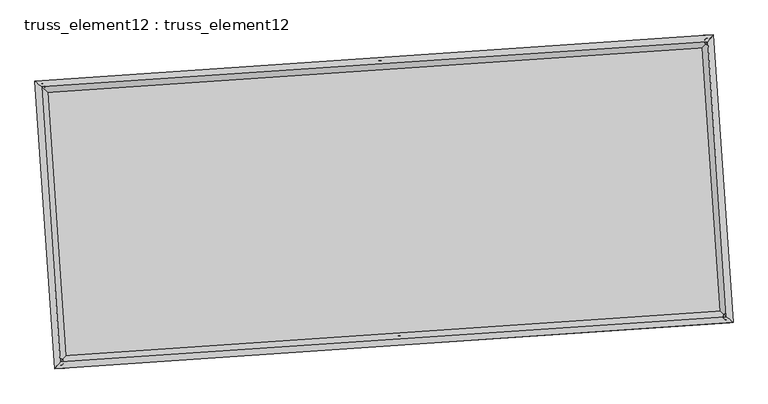
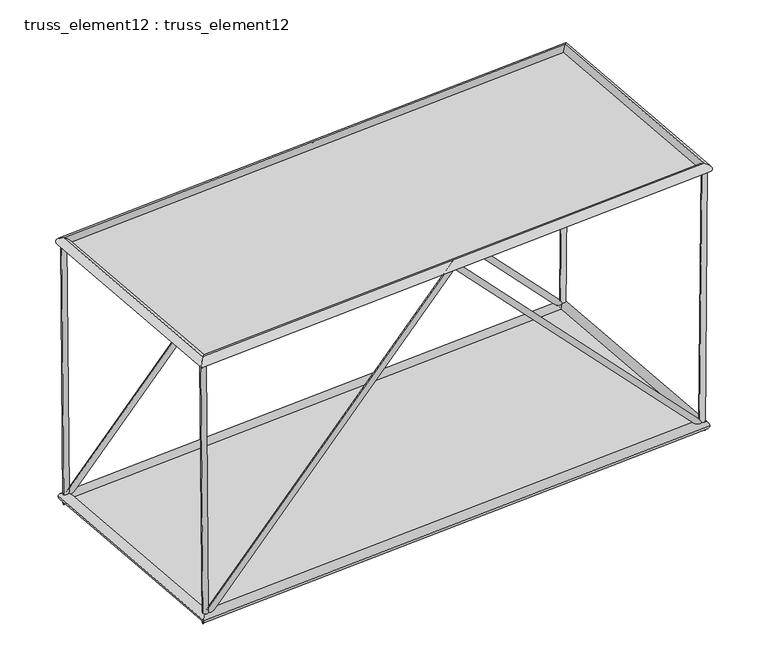
"""IFC4 building model written with IfcOpenShell, lengths in millimetres: plate geometry, truss_element12 : truss_element12."""

from ifc_helpers import new_model, si_unit, frame, origin, origin_with_axes, place, context, project, spatial, polyline, circle_curve, ellipse_curve, outline, extrude, source, transform, mapped, element, save
from ifc_brep_helpers import plane_surface, cylinder_surface, advanced_brep


def truss_element12_truss_element12_a0b56646(model_context):
    return source(origin(), model_context, "Body", "SolidModel", [
        advanced_brep(
        [(-3711.0240607, 2273.081801, 5000.2475381), (-3810.123175, 2259.720815, 4999.3258018), (-3666.0735064, 2276.1468084, 123.0270128), (-3762.9133765, 2262.9398717, -123.0270128), (1063.3254717, 2598.6265466, 5071.9126371), (1063.7795579, 2592.0537149, 4927.6678823), (5793.4932269, 2921.1587048, 123.0325352), (5891.2677501, 2921.2217837, -123.0325352), (5837.6808151, 2924.1716885, 5000.2468963), (5937.6764799, 2924.3862186, 4999.3408025)],
        [
            (0, 1, circle_curve(frame((-3760.5736179, 2266.401308, 4999.7866699), z_axis=(-0.009216035288574901, -0.0006284064129009009, 0.9999573339892758), x_axis=(-0.1336099520450236, 0.9910338088636684, -0.000608607998935612)), 50.0)),
            (1, 0, circle_curve(frame((-3760.5736179, 2266.401308, 4999.7866699), z_axis=(-0.009216035288574901, -0.0006284064129009009, 0.9999573339892758), x_axis=(-0.1336099520450236, 0.9910338088636684, -0.000608607998935612)), 50.0)),
            (0, 2),
            (2, 3, ellipse_curve(frame((-3714.4934414, 2269.54334, 0.0), z_axis=(-0.9275008521416528, -0.06324275734672205, 0.3684325215282871), x_axis=(0.36757900930277176, 0.025063815345724785, 0.9296544933900488)), 132.6244381, 50.0)),
            (3, 1),
            (3, 2, ellipse_curve(frame((-3714.4934414, 2269.54334, 0.0), z_axis=(-0.9275008521416528, -0.06324275734672205, 0.3684325215282871), x_axis=(0.36757900930277176, 0.025063815345724785, 0.9296544933900488)), 132.6244381, 50.0)),
            (2, 4),
            (4, 5, ellipse_curve(frame((1063.5525148, 2595.3401308, 4999.7902597), z_axis=(-0.9976833952413824, -0.06802823817186877, -4.08761425662505e-05), x_axis=(4.0781448733720234e-05, 2.7807319673914647e-06, -0.9999999991645705)), 72.2794243, 50.0)),
            (5, 3),
            (5, 4, ellipse_curve(frame((1063.5525148, 2595.3401308, 4999.7902597), z_axis=(-0.9976833952413824, -0.06802823817186877, -4.08761425662505e-05), x_axis=(4.0781448733720234e-05, 2.7807319673914647e-06, -0.9999999991645705)), 72.2794243, 50.0)),
            (4, 6),
            (6, 7, ellipse_curve(frame((5842.3804885, 2921.1902443, 0.0), z_axis=(-0.9274570070583223, -0.06323976771715853, -0.36854339206869385), x_axis=(-0.3676896230000489, -0.025071357673265647, 0.9296105464991785)), 132.6366613, 50.0)),
            (7, 5),
            (7, 6, ellipse_curve(frame((5842.3804885, 2921.1902443, 0.0), z_axis=(-0.9274570070583223, -0.06323976771715853, -0.36854339206869385), x_axis=(-0.3676896230000489, -0.025071357673265647, 0.9296105464991785)), 132.6366613, 50.0)),
            (8, 9, circle_curve(frame((5887.6786475, 2924.2789535, 4999.7938494), z_axis=(0.009059631795654766, 0.0006177418532581219, 0.9999587698834037), x_axis=(-0.0021508100122614596, 0.9999975080358999, -0.0005982794342249342)), 50.0)),
            (9, 8, circle_curve(frame((5887.6786475, 2924.2789535, 4999.7938494), z_axis=(0.009059631795654766, 0.0006177418532581219, 0.9999587698834037), x_axis=(-0.0021508100122614596, 0.9999975080358999, -0.0005982794342249342)), 50.0)),
            (6, 8),
            (9, 7),
        ],
        [
            plane_surface(frame((-3760.5736179, 2316.4012981, 4999.8180916), z_axis=(-0.009216035288575345, -0.0006284064128996167, 0.9999573339892759), x_axis=(0.9999575314449909, -5.791661640053289e-06, 0.009216033468739223))),
            cylinder_surface(frame((-3760.5736179, 2266.401308, 4999.7866699), z_axis=(-0.009216035288574901, -0.0006284064129009009, 0.9999573339892758), x_axis=(-0.1336099520450236, 0.9910338088636684, -0.000608607998935612)), 50.0),
            cylinder_surface(frame((-3714.4934414, 2269.54334, 0.0), z_axis=(-0.690127815089705, -0.047057192289536795, -0.7221559523353218), x_axis=(-0.020411436034741562, 0.9987523853625653, -0.04557462025717426)), 50.0),
            cylinder_surface(frame((1063.5525148, 2595.3401308, 4999.7902597), z_axis=(-0.6901867139153389, -0.04706120837656576, 0.722099399391028), x_axis=(-0.11534570305050372, 0.9922791785736945, -0.04557850981437397)), 50.0),
            plane_surface(frame((5887.6786475, 2874.2789631, 4999.8247378), z_axis=(0.009059631795653693, 0.0006177418532570572, 0.9999587698834038), x_axis=(0.9999589606937513, -5.596743422486847e-06, -0.009059630066911253))),
            cylinder_surface(frame((5842.3804885, 2921.1902443, 0.0), z_axis=(-0.009059631795654766, -0.0006177418532581219, -0.9999587698834037), x_axis=(-0.0021508100122614596, 0.9999975080358999, -0.0005982794342249342)), 50.0),
        ],
        [
            (0, [[1, 2]]),
            (1, [[-1, 3, 4, 5]]),
            (1, [[-2, -5, 6, -3]]),
            (2, [[-4, 7, 8, 9]]),
            (2, [[-6, -9, 10, -7]]),
            (3, [[-8, 11, 12, 13]]),
            (3, [[-10, -13, 14, -11]]),
            (4, [[15, 16]]),
            (5, [[-12, 17, -16, 18]]),
            (5, [[-14, -18, -15, -17]]),
        ],
    ),
        advanced_brep(
        [(-3438.9111078, -1717.6517833, 5000.2475381), (-3538.0102221, -1731.0127693, 4999.3258018), (-3393.9605535, -1714.5867759, 123.0270128), (-3490.8004235, -1727.7937126, -123.0270128), (1335.4384246, -1392.1070377, 5071.9126371), (1335.8925109, -1398.6798694, 4927.6678823), (6065.6061799, -1069.5748795, 123.0325352), (6163.380703, -1069.5118006, -123.0325352), (6109.793768, -1066.5618958, 5000.2468963), (6209.7894328, -1066.3473657, 4999.3408025)],
        [
            (0, 1, circle_curve(frame((-3488.4606649, -1724.3322763, 4999.7866699), z_axis=(-0.009216035288574948, -0.0006284064129009378, 0.9999573339892759), x_axis=(-0.13360995204502385, 0.9910338088636685, -0.0006086079989355841)), 50.0)),
            (1, 0, circle_curve(frame((-3488.4606649, -1724.3322763, 4999.7866699), z_axis=(-0.009216035288574948, -0.0006284064129009378, 0.9999573339892759), x_axis=(-0.13360995204502385, 0.9910338088636685, -0.0006086079989355841)), 50.0)),
            (0, 2),
            (2, 3, ellipse_curve(frame((-3442.3804885, -1721.1902443, 0.0), z_axis=(-0.9275008521416527, -0.06324275734672215, 0.368432521528287), x_axis=(0.36757900930277154, 0.02506381534572478, 0.9296544933900488)), 132.6244381, 50.0)),
            (3, 1),
            (3, 2, ellipse_curve(frame((-3442.3804885, -1721.1902443, 0.0), z_axis=(-0.9275008521416527, -0.06324275734672215, 0.368432521528287), x_axis=(0.36757900930277154, 0.02506381534572478, 0.9296544933900488)), 132.6244381, 50.0)),
            (2, 4),
            (4, 5, ellipse_curve(frame((1335.6654677, -1395.3934535, 4999.7902597), z_axis=(-0.9976833952413824, -0.06802823817186873, -4.08761425658493e-05), x_axis=(4.078144873325896e-05, 2.7807319672761547e-06, -0.9999999991645705)), 72.2794243, 50.0)),
            (5, 3),
            (5, 4, ellipse_curve(frame((1335.6654677, -1395.3934535, 4999.7902597), z_axis=(-0.9976833952413824, -0.06802823817186873, -4.08761425658493e-05), x_axis=(4.078144873325896e-05, 2.7807319672761547e-06, -0.9999999991645705)), 72.2794243, 50.0)),
            (4, 6),
            (6, 7, ellipse_curve(frame((6114.4934414, -1069.54334, 0.0), z_axis=(-0.9274570070583223, -0.06323976771715835, -0.3685433920686936), x_axis=(-0.3676896230000487, -0.02507135767326561, 0.9296105464991784)), 132.6366613, 50.0)),
            (7, 5),
            (7, 6, ellipse_curve(frame((6114.4934414, -1069.54334, 0.0), z_axis=(-0.9274570070583223, -0.06323976771715835, -0.3685433920686936), x_axis=(-0.3676896230000487, -0.02507135767326561, 0.9296105464991784)), 132.6366613, 50.0)),
            (8, 9, circle_curve(frame((6159.7916004, -1066.4546308, 4999.7938494), z_axis=(0.00905963179565426, 0.0006177418532580408, 0.9999587698834038), x_axis=(-0.0021508100122610767, 0.9999975080359, -0.0005982794342248575)), 50.0)),
            (9, 8, circle_curve(frame((6159.7916004, -1066.4546308, 4999.7938494), z_axis=(0.00905963179565426, 0.0006177418532580408, 0.9999587698834038), x_axis=(-0.0021508100122610767, 0.9999975080359, -0.0005982794342248575)), 50.0)),
            (6, 8),
            (9, 7),
        ],
        [
            plane_surface(frame((-3488.4606649, -1674.3322862, 4999.8180916), z_axis=(-0.009216035288575345, -0.0006284064128996218, 0.9999573339892759), x_axis=(0.9999575314449909, -5.791661640053289e-06, 0.009216033468739223))),
            cylinder_surface(frame((-3488.4606649, -1724.3322763, 4999.7866699), z_axis=(-0.009216035288574948, -0.0006284064129009378, 0.9999573339892759), x_axis=(-0.13360995204502385, 0.9910338088636685, -0.0006086079989355841)), 50.0),
            cylinder_surface(frame((-3442.3804885, -1721.1902443, 0.0), z_axis=(-0.6901278150897046, -0.0470571922895368, -0.7221559523353221), x_axis=(-0.020411436034741513, 0.9987523853625653, -0.0455746202571743)), 50.0),
            cylinder_surface(frame((1335.6654677, -1395.3934535, 4999.7902597), z_axis=(-0.6901867139153381, -0.047061208376565626, 0.722099399391029), x_axis=(-0.11534570305050376, 0.9922791785736946, -0.04557850981437398)), 50.0),
            plane_surface(frame((6159.7916004, -1116.4546212, 4999.8247378), z_axis=(0.009059631795653693, 0.0006177418532570623, 0.9999587698834038), x_axis=(0.9999589606937513, -5.5967434215986685e-06, -0.009059630066911253))),
            cylinder_surface(frame((6114.4934414, -1069.54334, 0.0), z_axis=(-0.00905963179565426, -0.0006177418532580408, -0.9999587698834038), x_axis=(-0.0021508100122610767, 0.9999975080359, -0.0005982794342248575)), 50.0),
        ],
        [
            (0, [[1, 2]]),
            (1, [[-1, 3, 4, 5]]),
            (1, [[-2, -5, 6, -3]]),
            (2, [[-4, 7, 8, 9]]),
            (2, [[-6, -9, 10, -7]]),
            (3, [[-8, 11, 12, 13]]),
            (3, [[-10, -13, 14, -11]]),
            (4, [[15, 16]]),
            (5, [[-12, 17, -16, 18]]),
            (5, [[-14, -18, -15, -17]]),
        ],
    ),
        advanced_brep(
        [(-3488.4587742, -1724.3301808, 4909.78667), (-3488.4625557, -1724.3343719, 5089.7866699), (-3760.5757755, 2266.4031275, 5089.7866699), (-3760.5714602, 2266.3994885, 4909.78667), (5887.6804049, 2924.28104, 5089.7938494), (5887.6768901, 2924.2768671, 4909.7938494), (6159.7936247, -1066.4564594, 5089.7938494), (6159.789576, -1066.4528022, 4909.7938494)],
        [
            (0, 1, ellipse_curve(frame((-3488.4606649, -1724.3322763, 4999.7866699), z_axis=(-0.7535719234052628, 0.6573654662780949, -5.249543305220569e-07), x_axis=(-0.6573654662778873, -0.753571923405444, -5.249543243964657e-07)), 127.2792206, 90.0)),
            (1, 2),
            (2, 3, ellipse_curve(frame((-3760.5736179, 2266.401308, 4999.7866699), z_axis=(-0.657365466277887, -0.7535719234054442, -5.249543256633394e-07), x_axis=(0.7535719234052629, -0.6573654662780947, 5.249543317889309e-07)), 127.2792206, 90.0)),
            (3, 0),
            (1, 0, ellipse_curve(frame((-3488.4606649, -1724.3322763, 4999.7866699), z_axis=(-0.7535719234052628, 0.6573654662780949, -5.249543305220569e-07), x_axis=(-0.6573654662778873, -0.753571923405444, -5.249543243964657e-07)), 127.2792206, 90.0)),
            (3, 2, ellipse_curve(frame((-3760.5736179, 2266.401308, 4999.7866699), z_axis=(-0.657365466277887, -0.7535719234054442, -5.249543256633394e-07), x_axis=(0.7535719234052629, -0.6573654662780947, 5.249543317889309e-07)), 127.2792206, 90.0)),
            (2, 4),
            (4, 5, ellipse_curve(frame((5887.6786475, 2924.2789535, 4999.7938494), z_axis=(-0.7535719234052615, 0.6573654662780964, -5.249543287261489e-07), x_axis=(-0.6573654662778888, -0.7535719234054427, -5.249543287261216e-07)), 127.2792206, 90.0)),
            (5, 3),
            (5, 4, ellipse_curve(frame((5887.6786475, 2924.2789535, 4999.7938494), z_axis=(-0.7535719234052615, 0.6573654662780964, -5.249543287261489e-07), x_axis=(-0.6573654662778888, -0.7535719234054427, -5.249543287261216e-07)), 127.2792206, 90.0)),
            (4, 6),
            (6, 7, ellipse_curve(frame((6159.7916004, -1066.4546308, 4999.7938494), z_axis=(0.6573654662778889, 0.7535719234054424, 5.249543274592477e-07), x_axis=(-0.7535719234052612, 0.6573654662780967, -5.249543274592748e-07)), 127.2792206, 90.0)),
            (7, 5),
            (7, 6, ellipse_curve(frame((6159.7916004, -1066.4546308, 4999.7938494), z_axis=(0.6573654662778889, 0.7535719234054424, 5.249543274592477e-07), x_axis=(-0.7535719234052612, 0.6573654662780967, -5.249543274592748e-07)), 127.2792206, 90.0)),
            (6, 1),
            (0, 7),
        ],
        [
            cylinder_surface(frame((-3488.4606649, -1724.3322763, 4999.7866699), z_axis=(0.0680282382287011, -0.9976833960748765, 0.0), x_axis=(-0.9976833958213657, -0.06802823821141515, -2.2543273994709853e-05)), 90.0),
            cylinder_surface(frame((-3760.5736179, 2266.401308, 4999.7866699), z_axis=(-0.9976833960746018, -0.068028238228681, -7.423975313109646e-07), x_axis=(-0.06802823819638615, 0.9976833958388892, -2.1800876467906795e-05)), 90.0),
            cylinder_surface(frame((5887.6786475, 2924.2789535, 4999.7938494), z_axis=(-0.06802823822869654, 0.997683396074877, 0.0), x_axis=(0.9976833958536608, 0.06802823821361265, -2.105847893677226e-05)), 90.0),
            cylinder_surface(frame((6159.7916004, -1066.4546308, 4999.7938494), z_axis=(0.9976833960746019, 0.06802823822868047, 7.423975295193343e-07), x_axis=(0.06802823822868047, -0.9976833958366871, -2.180087646611519e-05)), 90.0),
        ],
        [
            (0, [[1, 2, 3, 4]]),
            (0, [[5, -4, 6, -2]]),
            (1, [[-3, 7, 8, 9]]),
            (1, [[-6, -9, 10, -7]]),
            (2, [[-8, 11, 12, 13]]),
            (2, [[-10, -13, 14, -11]]),
            (3, [[-12, 15, -1, 16]]),
            (3, [[-14, -16, -5, -15]]),
        ],
    ),
        advanced_brep(
        [(-3358.7115243, -1625.2761972, 0.0), (-3526.0494527, -1817.1042913, 0.0), (-3810.4074885, 2353.2123043, 0.0), (-3618.5793943, 2185.8743758, 0.0), (5926.0494527, 3017.1042913, 0.0), (5758.7115243, 2825.2761972, 0.0), (6210.4074885, -1153.2123043, 0.0), (6018.5793943, -985.8743758, 0.0)],
        [
            (0, 1, ellipse_curve(frame((-3442.3804885, -1721.1902443, 0.0), z_axis=(-0.7535719234054586, 0.6573654662780799, 0.0), x_axis=(-0.65736546627808, -0.7535719234054586, 0.0)), 127.2792206, 90.0)),
            (1, 2),
            (2, 3, ellipse_curve(frame((-3714.4934414, 2269.54334, 0.0), z_axis=(-0.6573654662780798, -0.7535719234054588, 0.0), x_axis=(0.7535719234054588, -0.6573654662780799, 0.0)), 127.2792206, 90.0)),
            (3, 0),
            (1, 0, ellipse_curve(frame((-3442.3804885, -1721.1902443, 0.0), z_axis=(-0.7535719234054586, 0.6573654662780799, 0.0), x_axis=(-0.65736546627808, -0.7535719234054586, 0.0)), 127.2792206, 90.0)),
            (3, 2, ellipse_curve(frame((-3714.4934414, 2269.54334, 0.0), z_axis=(-0.6573654662780798, -0.7535719234054588, 0.0), x_axis=(0.7535719234054588, -0.6573654662780799, 0.0)), 127.2792206, 90.0)),
            (2, 4),
            (4, 5, ellipse_curve(frame((5842.3804885, 2921.1902443, 0.0), z_axis=(-0.7535719234054573, 0.6573654662780815, 0.0), x_axis=(-0.6573654662780816, -0.7535719234054574, 0.0)), 127.2792206, 90.0)),
            (5, 3),
            (5, 4, ellipse_curve(frame((5842.3804885, 2921.1902443, 0.0), z_axis=(-0.7535719234054573, 0.6573654662780815, 0.0), x_axis=(-0.6573654662780816, -0.7535719234054574, 0.0)), 127.2792206, 90.0)),
            (4, 6),
            (6, 7, ellipse_curve(frame((6114.4934414, -1069.54334, 0.0), z_axis=(0.6573654662780818, 0.7535719234054571, 0.0), x_axis=(-0.7535719234054571, 0.6573654662780818, 0.0)), 127.2792206, 90.0)),
            (7, 5),
            (7, 6, ellipse_curve(frame((6114.4934414, -1069.54334, 0.0), z_axis=(0.6573654662780818, 0.7535719234054571, 0.0), x_axis=(-0.7535719234054571, 0.6573654662780818, 0.0)), 127.2792206, 90.0)),
            (6, 1),
            (0, 7),
        ],
        [
            cylinder_surface(frame((-3442.3804885, -1721.1902443, 0.0), z_axis=(0.06802823822870321, -0.9976833960748764, 0.0), x_axis=(-0.9976833960748764, -0.06802823822870321, 0.0)), 90.0),
            cylinder_surface(frame((-3714.4934414, 2269.54334, 0.0), z_axis=(-0.9976833960748765, -0.06802823822870187, 0.0), x_axis=(-0.06802823822870187, 0.9976833960748765, 0.0)), 90.0),
            cylinder_surface(frame((5842.3804885, 2921.1902443, 0.0), z_axis=(-0.06802823822869863, 0.9976833960748768, 0.0), x_axis=(0.9976833960748768, 0.06802823822869863, 0.0)), 90.0),
            cylinder_surface(frame((6114.4934414, -1069.54334, 0.0), z_axis=(0.9976833960748768, 0.06802823822870137, 0.0), x_axis=(0.06802823822870137, -0.9976833960748768, 0.0)), 90.0),
        ],
        [
            (0, [[1, 2, 3, 4]]),
            (0, [[5, -4, 6, -2]]),
            (1, [[-3, 7, 8, 9]]),
            (1, [[-6, -9, 10, -7]]),
            (2, [[-8, 11, 12, 13]]),
            (2, [[-10, -13, 14, -11]]),
            (3, [[-12, 15, -1, 16]]),
            (3, [[-14, -16, -5, -15]]),
        ],
    ),
        extrude(outline(polyline([(-3442.3804885, -1721.1902443), (-3714.4934414, 2269.54334), (5842.3804885, 2921.1902443), (6114.4934414, -1069.54334), (-3442.3804885, -1721.1902443)])), origin_with_axes(), (0.0, 0.0, 1.0), 20.0),
        extrude(outline(polyline([(-2000.0, 4835.3276717), (2000.0, 4835.3276718), (2000.0, -4835.3276717), (-2000.0, -4835.3276717), (-2000.0, 4835.3276717)])), frame((1199.6089913, 599.9733386, 4999.7902597), z_axis=(-7.406776905705705e-07, -5.0503991798987605e-08, 0.9999999999997244), x_axis=(-0.0680282382287028, 0.9976833960748765, 0.0)), (0.0, 0.0, 1.0), 20.0),
    ])


if __name__ == "__main__":
    model = new_model("IFC4")
    model_context = context("Model", 3, world=origin())
    ifc_project = project(units=[si_unit("LENGTHUNIT", "METRE", prefix="MILLI")], contexts=[model_context])
    site = spatial("IfcSite", under=ifc_project)
    building = spatial("IfcBuilding", under=site)
    placement = place(None, origin())
    truss_element12_truss_element12_shape = truss_element12_truss_element12_a0b56646(model_context)
    element("IfcPlate", 1, ObjectType="truss_element12 : truss_element12", at=placement, inside=building, context=model_context, shape_type="MappedRepresentation", body=[
        mapped(truss_element12_truss_element12_shape, transform((0.0, 0.0, 0.0), x_axis=(1.0, 0.0, 0.0), y_axis=(0.0, 1.0, 0.0), z_axis=(0.0, 0.0, 1.0))),
    ])
    save(model, "model.ifc")

# Revit data of these elements
# Type "truss_element12 : truss_element12"
#   steellbar1 = 90 mm
#   steelbar2 = 50 mm
#   offset1 = 5000 mm
#   M = Default Roof
# Element 1 (IfcPlate, "truss_element12 : truss_element12")
#   Materials on its faces: "Default Roof"
# Materials
#   "Default Roof": class "Miscellaneous", colour RGB 0 127 0, transparency 0, Comments = "Rendering appearance not upgraded Rendering appearance not upgraded ", Cost = 0
